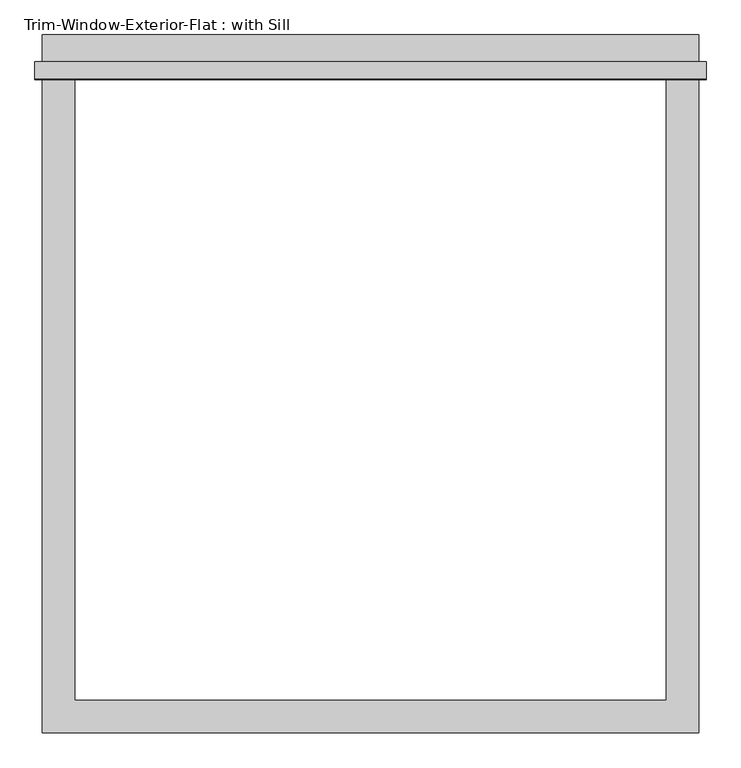
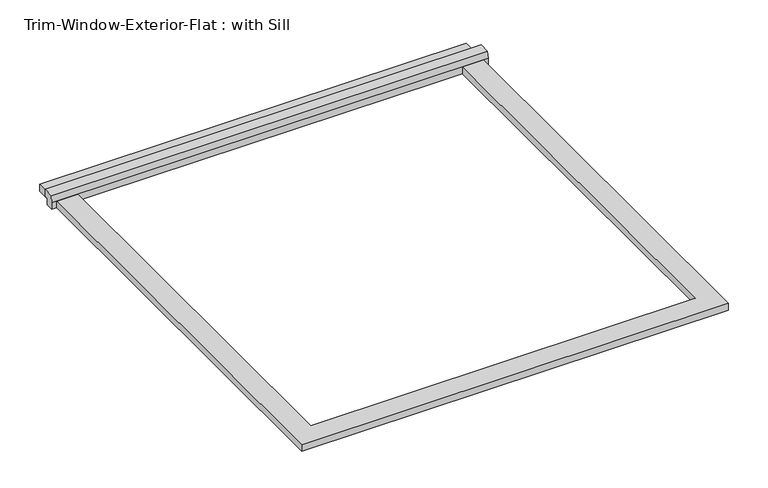
"""IFC4 building model written with IfcOpenShell, lengths in millimetres: proxy geometry, Trim-Window-Exterior-Flat : with Sill."""

from ifc_helpers import new_model, si_unit, frame, origin, origin_with_axes, place, context, project, spatial, polyline, outline, extrude, source, transform, mapped, element, save


def trim_window_exterior_flat_with_sill_26b0c1ac(model_context):
    return source(origin(), model_context, "Body", "SweptSolid", [
        extrude(outline(polyline([(577.85, 1114.3823709), (-577.85, 1114.3823709), (-577.85, 1171.5323709), (577.85, 1171.5323709), (577.85, 1114.3823709)])), origin_with_axes(), (0.0, 0.0, 1.0), 19.05),
        extrude(outline(polyline([(1123.95, 38.1), (1123.95, 19.05), (1114.3823709, 19.05), (1114.3823709, 0.0), (1092.2, 0.0), (1092.2, 19.05), (1094.6580645, 38.1), (1123.95, 38.1)])), frame((-590.55, 0.0, 0.0), z_axis=(1.0, 0.0, 0.0), x_axis=(0.0, 1.0, 0.0)), (0.0, 0.0, 1.0), 1181.1),
        extrude(outline(polyline([(-577.85, -57.15), (-577.85, 1092.2), (-520.7, 1092.2), (-520.7, 0.0), (520.7, 0.0), (520.7, 1092.2), (577.85, 1092.2), (577.85, -57.15), (-577.85, -57.15)])), origin_with_axes(), (0.0, 0.0, 1.0), 19.05),
    ])


if __name__ == "__main__":
    model = new_model("IFC4")
    model_context = context("Model", 3, world=origin())
    ifc_project = project(units=[si_unit("LENGTHUNIT", "METRE", prefix="MILLI")], contexts=[model_context])
    site = spatial("IfcSite", under=ifc_project)
    building = spatial("IfcBuilding", under=site)
    placement = place(None, origin())
    trim_window_exterior_flat_with_sill_shape = trim_window_exterior_flat_with_sill_26b0c1ac(model_context)
    element("IfcBuildingElementProxy", 1, Name="Trim-Window-Exterior-Flat : with Sill", ObjectType="Trim-Window-Exterior-Flat : with Sill", at=placement, inside=building, context=model_context, shape_type="MappedRepresentation", body=[
        mapped(trim_window_exterior_flat_with_sill_shape, transform((0.0, 0.0, 0.0), x_axis=(1.0, 0.0, 0.0), y_axis=(0.0, 1.0, 0.0), z_axis=(0.0, 0.0, 1.0))),
    ])
    save(model, "model.ifc")

# Revit data of these elements
# Type "Trim-Window-Exterior-Flat : with Sill"
#   Trim Width = 0' - 2 1/4"
#   Trim Thickness_Picture Frame = 0' - 1 1/4"
#   Trim Thickness_with Sill = 0' - 0 3/4"
#   Sill Thickness = 0' - 1 1/4"
#   Opening Width [instance default] = 2' - 0"
#   Opening Height [instance default] = 3' - 0"
#   Default Elevation = 4' - 0"
#   Sill = yes
#   Picture Frame = no
#   Trim Material [instance default] = none
# Element 1 (IfcBuildingElementProxy, "Trim-Window-Exterior-Flat : with Sill")
#   Opening Width = 3' - 5"
#   Opening Height = 3' - 7"
#   Trim Material = Clad - White
#   Materials on its faces: "Clad - White"
# Materials
#   "Clad - White": class "Wood", colour RGB 242 242 238, transparency 0, Cost = 0
